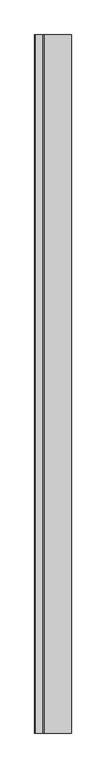
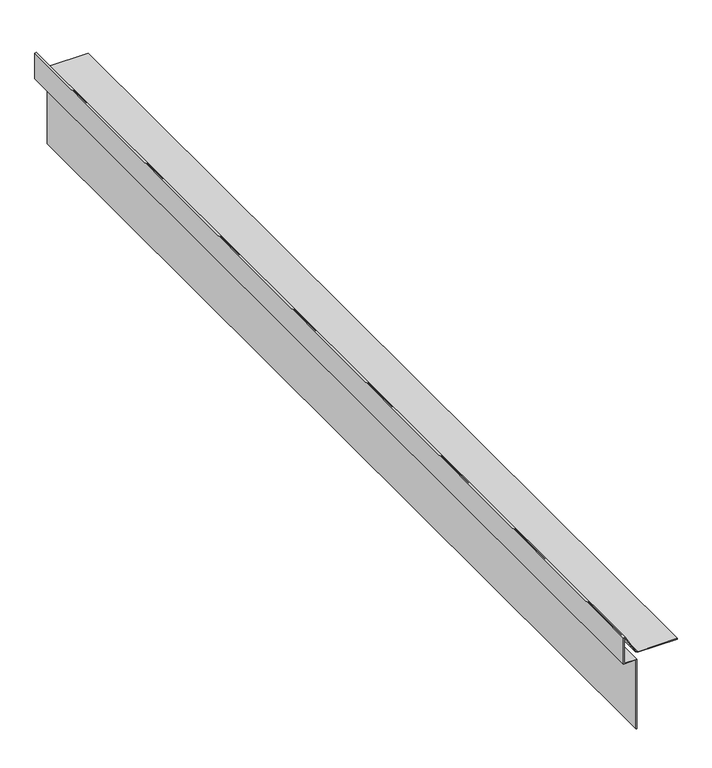
"""IFC4 building model written with IfcOpenShell, lengths in millimetres: proxy geometry, GRAVEL STOP11:GRAVEL STOP002:299934 : GRAVEL STOP11:GRAVEL STOP002:299934."""

from ifc_helpers import new_model, si_unit, frame, origin, place, context, project, spatial, polyline, outline, extrude, source, transform, mapped, element, save


def generic_models_d8596f44(model_context):
    return source(origin(), model_context, "Body", "SweptSolid", [
        extrude(outline(polyline([(40259.5408757, -237.2292147), (40295.3431515, -257.8996682), (40294.5307525, -260.9315826), (40240.9633674, -260.9315826), (40240.9633674, -236.591845), (40097.9858473, -236.591845), (40097.9858473, -235.180734), (40242.3744784, -235.180734), (40242.3744784, -259.5204716), (40293.447969, -259.5204716), (40293.699878, -258.5803344), (40258.5078708, -238.2622196), (40255.9633674, -233.8550105), (40255.9633674, -156.0189978), (40257.3744784, -156.0189978), (40257.3744784, -233.4769045), (40259.5408757, -237.2292147)])), frame((0.0, -774.5581162, 0.0), z_axis=(0.0, 1.0, 0.0), x_axis=(0.0, 0.0, 1.0)), (0.0, 0.0, 1.0), 2000.25),
    ])


if __name__ == "__main__":
    model = new_model("IFC4")
    model_context = context("Model", 3, world=origin())
    ifc_project = project(units=[si_unit("LENGTHUNIT", "METRE", prefix="MILLI")], contexts=[model_context])
    site = spatial("IfcSite", under=ifc_project)
    building = spatial("IfcBuilding", under=site)
    placement = place(None, origin())
    generic_models_shape = generic_models_d8596f44(model_context)
    element("IfcBuildingElementProxy", 1, Name="GRAVEL STOP11:GRAVEL STOP002:299934 : GRAVEL STOP11:GRAVEL STOP002:299934", ObjectType="GRAVEL STOP11:GRAVEL STOP002:299934 : GRAVEL STOP11:GRAVEL STOP002:299934", at=placement, inside=building, context=model_context, shape_type="MappedRepresentation", body=[
        mapped(generic_models_shape, transform((0.0, 0.0, 0.0), x_axis=(1.0, 0.0, 0.0), y_axis=(0.0, 1.0, 0.0), z_axis=(0.0, 0.0, 1.0))),
    ])
    save(model, "model.ifc")

# Revit data of these elements
# Type "GRAVEL STOP11:GRAVEL STOP002:299934 : GRAVEL STOP11:GRAVEL STOP002:299934"
#   NameOverride = "GRAVEL STOP11:GRAVEL STOP002:299934"
#   ObjectTypeOverride = "GRAVEL STOP11:GRAVEL STOP002"
#   Reference = "GRAVEL STOP002"
#   Category = "Generic Models"
#   Tag = "299934"
# Element 1 (IfcBuildingElementProxy, "GRAVEL STOP11:GRAVEL STOP002:299934 : GRAVEL STOP11:GRAVEL STOP002:299934")
#   Materials on its faces: "GRAVEL STOP REQUIRED WITH GRAVEL SURFACE SYSTEMS"
# Materials
#   "GRAVEL STOP REQUIRED WITH GRAVEL SURFACE SYSTEMS": class "Unassigned", colour RGB 170 170 127, transparency 0, Cost = 0
